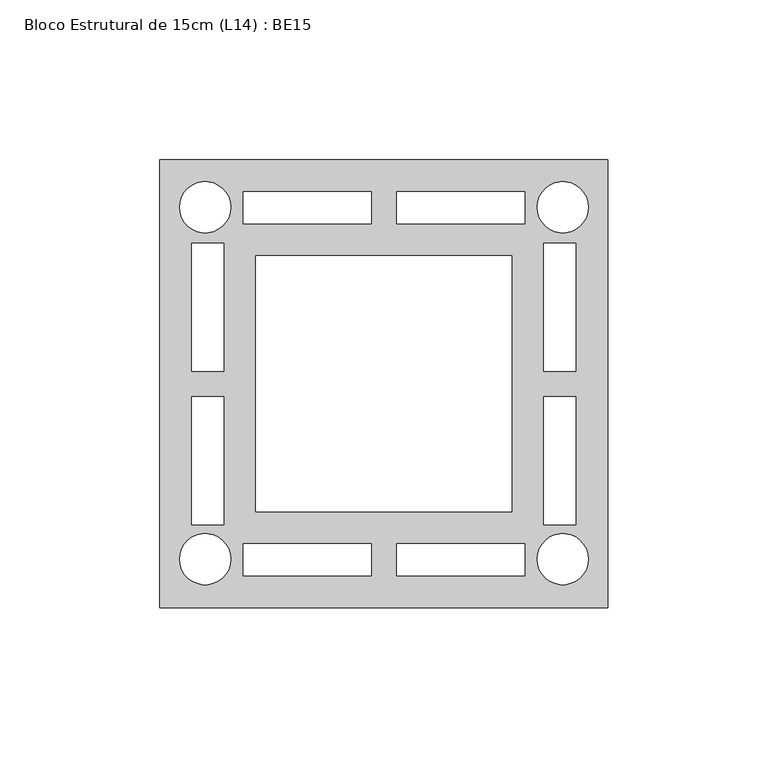
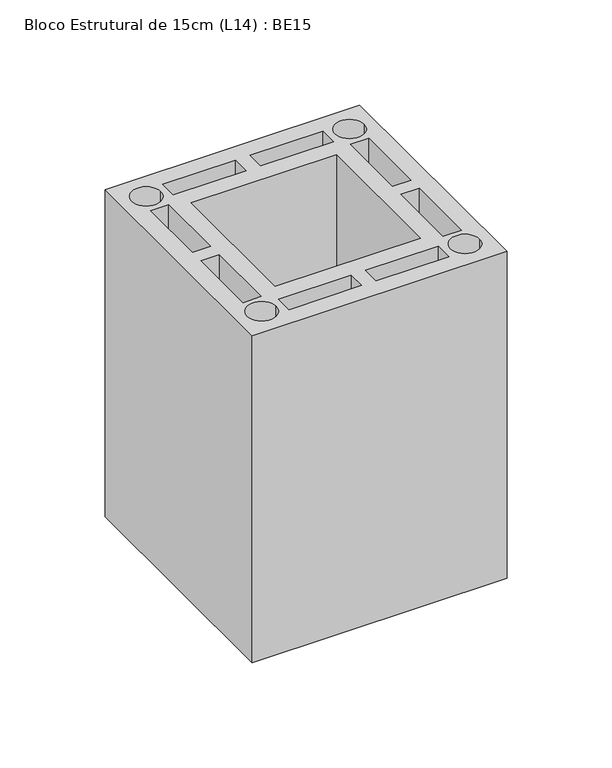
"""IFC4 building model written with IfcOpenShell, lengths in millimetres: proxy geometry, Bloco Estrutural de 15cm (L14) : BE15."""

from ifc_helpers import new_model, si_unit, point, frame_2d, origin, origin_with_axes, place, context, project, spatial, polyline, circle_curve, trimmed, segment, composite_curve, outline, extrude, source, transform, mapped, element, save


def bloco_estrutural_de_15cm_l14_be15_6fc3eb17(model_context):
    return source(origin(), model_context, "Body", "SweptSolid", [
        extrude(outline(polyline([(0.0, -140.0), (0.0, 0.0), (140.0, 0.0), (140.0, -140.0), (0.0, -140.0)]), holes=[polyline([(30.0, -110.0), (110.0, -110.0), (110.0, -30.0), (30.0, -30.0), (30.0, -110.0)]), composite_curve([segment(trimmed(circle_curve(frame_2d((14.1087523, -124.7509514)), 8.0), [point((6.1087523, -124.7509514))], [point((22.1087523, -124.7509514))], True, "CARTESIAN"), True, "CONTINUOUS"), segment(trimmed(circle_curve(frame_2d((14.1087523, -124.7509514)), 8.0), [point((22.1087523, -124.7509514))], [point((6.1087523, -124.7509514))], True, "CARTESIAN"), True, "CONTINUOUS")], self_intersect=False), composite_curve([segment(trimmed(circle_curve(frame_2d((14.1087523, -14.7509514)), 8.0), [point((6.1087523, -14.7509514))], [point((22.1087523, -14.7509514))], True, "CARTESIAN"), True, "CONTINUOUS"), segment(trimmed(circle_curve(frame_2d((14.1087523, -14.7509514)), 8.0), [point((22.1087523, -14.7509514))], [point((6.1087523, -14.7509514))], True, "CARTESIAN"), True, "CONTINUOUS")], self_intersect=False), polyline([(20.0, -66.0), (20.0, -26.0), (10.0, -26.0), (10.0, -66.0), (20.0, -66.0)]), polyline([(20.0, -74.0), (10.0, -74.0), (10.0, -114.0), (20.0, -114.0), (20.0, -74.0)]), composite_curve([segment(trimmed(circle_curve(frame_2d((125.8912477, -124.7509514)), 8.0), [point((133.8912477, -124.7509514))], [point((117.8912477, -124.7509514))], True, "CARTESIAN"), True, "CONTINUOUS"), segment(trimmed(circle_curve(frame_2d((125.8912477, -124.7509514)), 8.0), [point((117.8912477, -124.7509514))], [point((133.8912477, -124.7509514))], True, "CARTESIAN"), True, "CONTINUOUS")], self_intersect=False), composite_curve([segment(trimmed(circle_curve(frame_2d((125.8912477, -14.7509514)), 8.0), [point((133.8912477, -14.7509514))], [point((117.8912477, -14.7509514))], True, "CARTESIAN"), True, "CONTINUOUS"), segment(trimmed(circle_curve(frame_2d((125.8912477, -14.7509514)), 8.0), [point((117.8912477, -14.7509514))], [point((133.8912477, -14.7509514))], True, "CARTESIAN"), True, "CONTINUOUS")], self_intersect=False), polyline([(120.0, -66.0), (130.0, -66.0), (130.0, -26.0), (120.0, -26.0), (120.0, -66.0)]), polyline([(120.0, -74.0), (120.0, -114.0), (130.0, -114.0), (130.0, -74.0), (120.0, -74.0)]), polyline([(66.0, -120.0), (26.0, -120.0), (26.0, -130.0), (66.0, -130.0), (66.0, -120.0)]), polyline([(74.0, -120.0), (74.0, -130.0), (114.0, -130.0), (114.0, -120.0), (74.0, -120.0)]), polyline([(66.0, -20.0), (66.0, -10.0), (26.0, -10.0), (26.0, -20.0), (66.0, -20.0)]), polyline([(74.0, -20.0), (114.0, -20.0), (114.0, -10.0), (74.0, -10.0), (74.0, -20.0)])]), origin_with_axes(), (0.0, 0.0, 1.0), 190.0),
    ])


if __name__ == "__main__":
    model = new_model("IFC4")
    model_context = context("Model", 3, world=origin())
    ifc_project = project(units=[si_unit("LENGTHUNIT", "METRE", prefix="MILLI")], contexts=[model_context])
    site = spatial("IfcSite", under=ifc_project)
    building = spatial("IfcBuilding", under=site)
    placement = place(None, origin())
    bloco_estrutural_de_15cm_l14_be15_shape = bloco_estrutural_de_15cm_l14_be15_6fc3eb17(model_context)
    element("IfcBuildingElementProxy", 1, Name="Bloco Estrutural de 15cm (L14) : BE15", ObjectType="Bloco Estrutural de 15cm (L14) : BE15", at=placement, inside=building, context=model_context, shape_type="MappedRepresentation", body=[
        mapped(bloco_estrutural_de_15cm_l14_be15_shape, transform((0.0, 0.0, 0.0), x_axis=(1.0, 0.0, 0.0), y_axis=(0.0, 1.0, 0.0), z_axis=(0.0, 0.0, 1.0))),
    ])
    save(model, "model.ifc")

# Revit data of these elements
# Type "Bloco Estrutural de 15cm (L14) : BE15"
#   Material [instance default] = Blocos Cerâmicos
#   Default Elevation = 0
# Element 1 (IfcBuildingElementProxy, "Bloco Estrutural de 15cm (L14) : BE15")
#   Materials on its faces: "Blocos Cerâmicos"
# Materials
#   "Blocos Cerâmicos": class "Genérico", colour RGB 177 84 47, transparency 0, Cost = 0
